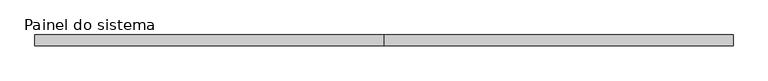
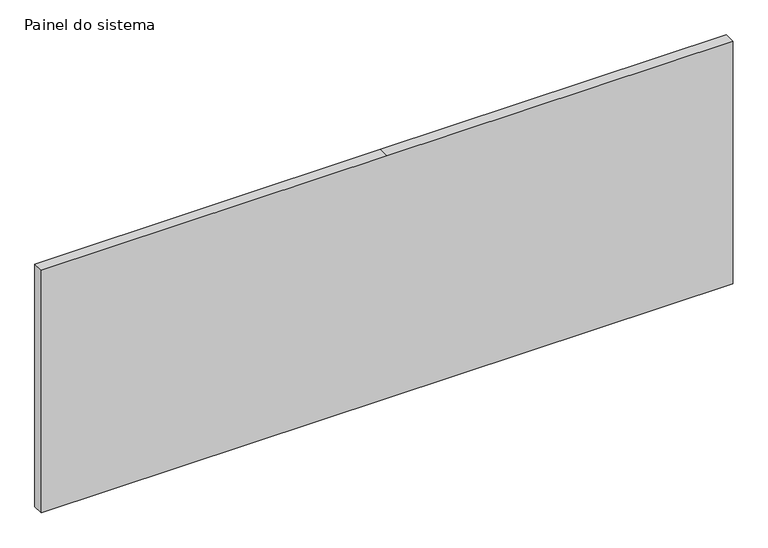
"""IFC4 building model written with IfcOpenShell, lengths in millimetres: plate geometry, Painel do sistema : Envidraçado."""

from ifc_helpers import new_model, si_unit, frame, origin, place, context, project, spatial, polyline, outline, extrude, source, transform, mapped, element, save


def painel_do_sistema_17e406c8(model_context):
    return source(origin(), model_context, "Body", "SweptSolid", [
        extrude(outline(polyline([(0.0, -795.9833332), (0.0, 0.0), (0.0, 795.9833332), (590.0, 795.9833332), (590.0, 0.0), (590.0, -795.9833332), (0.0, -795.9833332)])), frame((0.0, -49.5, 0.0), z_axis=(0.0, 1.0, 0.0), x_axis=(0.0, 0.0, 1.0)), (0.0, 0.0, 1.0), 25.0),
    ])


if __name__ == "__main__":
    model = new_model("IFC4")
    model_context = context("Model", 3, world=origin())
    ifc_project = project(units=[si_unit("LENGTHUNIT", "METRE", prefix="MILLI")], contexts=[model_context])
    site = spatial("IfcSite", under=ifc_project)
    building = spatial("IfcBuilding", under=site)
    placement = place(None, origin())
    painel_do_sistema_shape = painel_do_sistema_17e406c8(model_context)
    element("IfcPlate", 1, ObjectType="Painel do sistema : Envidraçado", at=placement, inside=building, context=model_context, shape_type="MappedRepresentation", body=[
        mapped(painel_do_sistema_shape, transform((0.0, 0.0, 0.0), x_axis=(1.0, 0.0, 0.0), y_axis=(0.0, 1.0, 0.0), z_axis=(0.0, 0.0, 1.0))),
    ])
    save(model, "model.ifc")

# Revit data of these elements
# Type "Painel do sistema : Envidraçado"
#   Construction Type Id = "GSP4R"
#   Analytic Construction = "Vidraça única Pilkington 1/8 pol"
#   Visual Light Transmittance = 0.9
#   Solar Heat Gain Coefficient = 0.86
#   Heat Transfer Coefficient (U) = 6.7069 W/(m²·K)
# Element 1 (IfcPlate, "Painel do sistema : Envidraçado")
#   Materials on its faces: ".VIDRO GENÉRICO"
# Materials
#   ".VIDRO GENÉRICO": class ".CC_VIDRO", colour RGB 0 128 192, transparency 0.9, Description = "Vidro comum", Cost = 0
